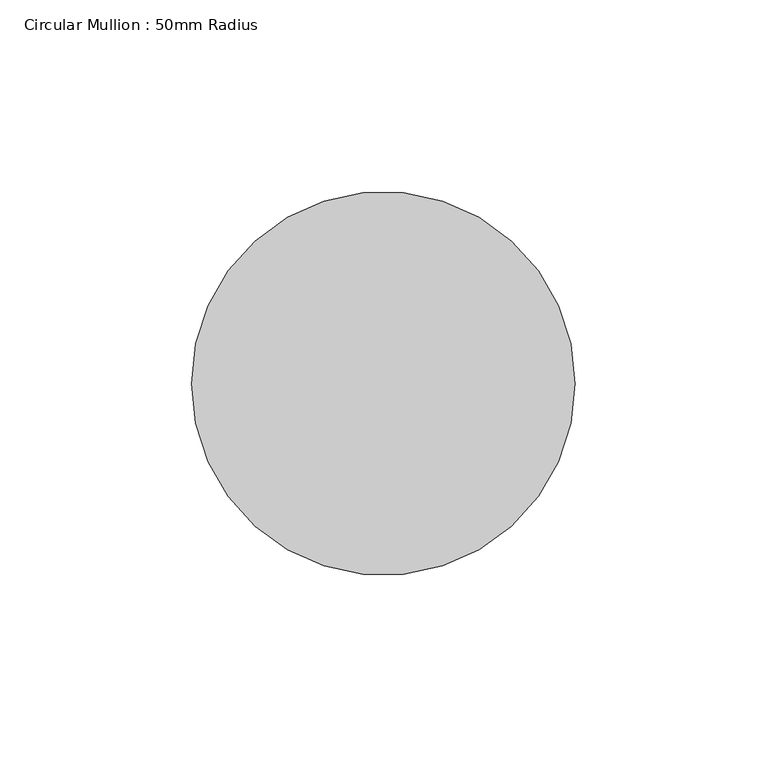
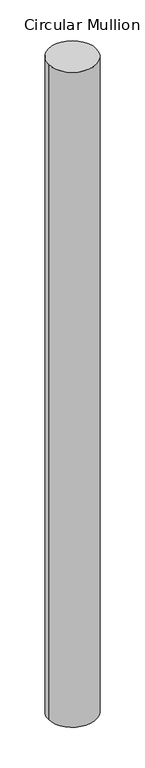
"""IFC4 building model written with IfcOpenShell, lengths in millimetres: member geometry, Circular Mullion : 50mm Radius."""

from ifc_helpers import new_model, si_unit, point, frame, origin, origin_2d, place, context, project, spatial, circle_curve, trimmed, segment, composite_curve, outline, extrude, source, transform, mapped, element, save


def circular_mullion_50mm_radius_b95fd494(model_context):
    return source(origin(), model_context, "Body", "SweptSolid", [
        extrude(outline(composite_curve([segment(trimmed(circle_curve(origin_2d(), 50.0), [point((50.0, 0.0))], [point((-50.0, 0.0))], False, "CARTESIAN"), True, "CONTINUOUS"), segment(trimmed(circle_curve(origin_2d(), 50.0), [point((-50.0, 0.0))], [point((50.0, 0.0))], False, "CARTESIAN"), True, "CONTINUOUS")], self_intersect=False)), frame((0.0, 0.0, -1448.7840928), z_axis=(0.0, 0.0, 1.0), x_axis=(1.0, 0.0, 0.0)), (0.0, 0.0, 1.0), 1448.7840928),
    ])


if __name__ == "__main__":
    model = new_model("IFC4")
    model_context = context("Model", 3, world=origin())
    ifc_project = project(units=[si_unit("LENGTHUNIT", "METRE", prefix="MILLI")], contexts=[model_context])
    site = spatial("IfcSite", under=ifc_project)
    building = spatial("IfcBuilding", under=site)
    placement = place(None, origin())
    circular_mullion_50mm_radius_shape = circular_mullion_50mm_radius_b95fd494(model_context)
    element("IfcMember", 1, ObjectType="Circular Mullion : 50mm Radius", at=placement, inside=building, context=model_context, shape_type="MappedRepresentation", body=[
        mapped(circular_mullion_50mm_radius_shape, transform((0.0, 0.0, 0.0), x_axis=(1.0, 0.0, 0.0), y_axis=(0.0, 1.0, 0.0), z_axis=(0.0, 0.0, 1.0))),
    ])
    save(model, "model.ifc")

# Revit data of these elements
# Type "Circular Mullion : 50mm Radius"
#   built-in parameter 1007350 = 0.164042 (stored number, unit not read)
# Element 1 (IfcMember, "Circular Mullion : 50mm Radius")
#   Materials on its faces: "Aluminium"
# Materials
#   "Aluminium": class "Metal", colour RGB 247 247 247, transparency 0, Description = "Aluminium 6061", Cost = 0
